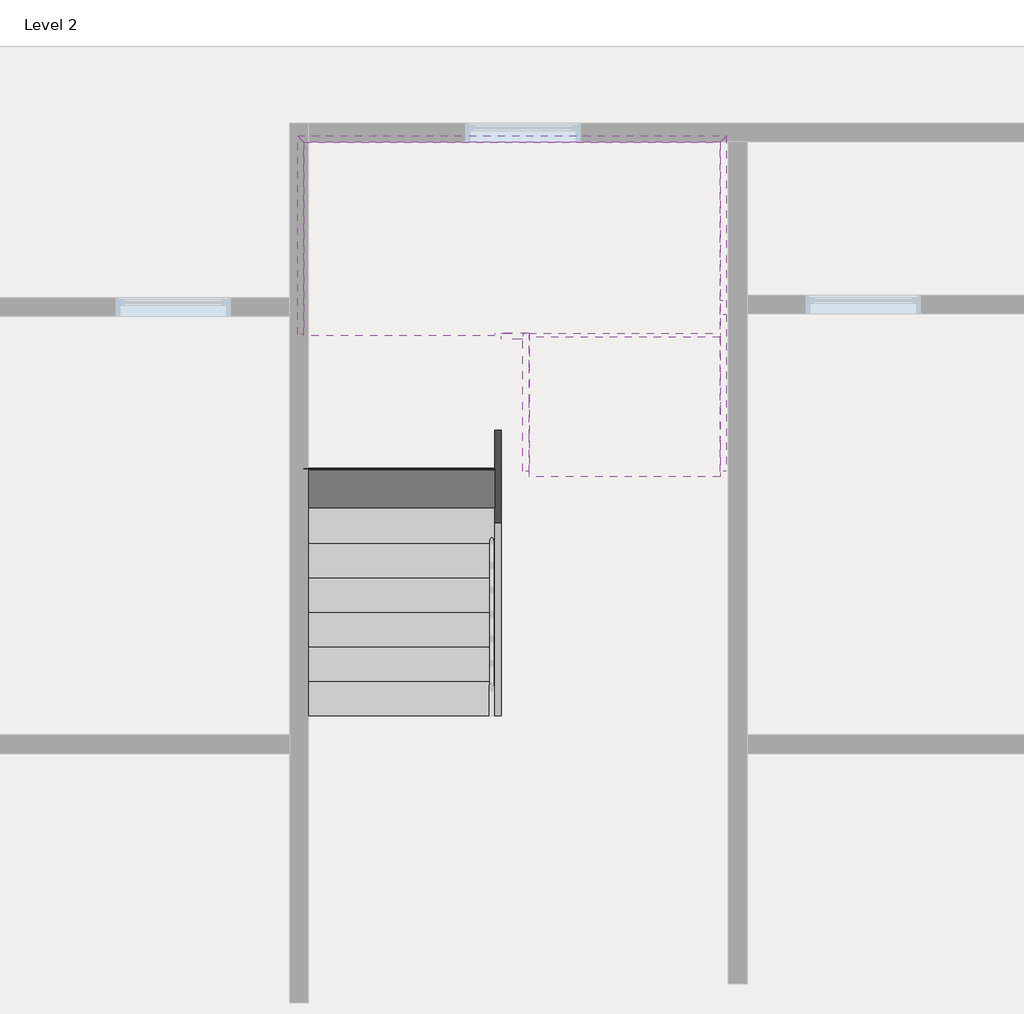
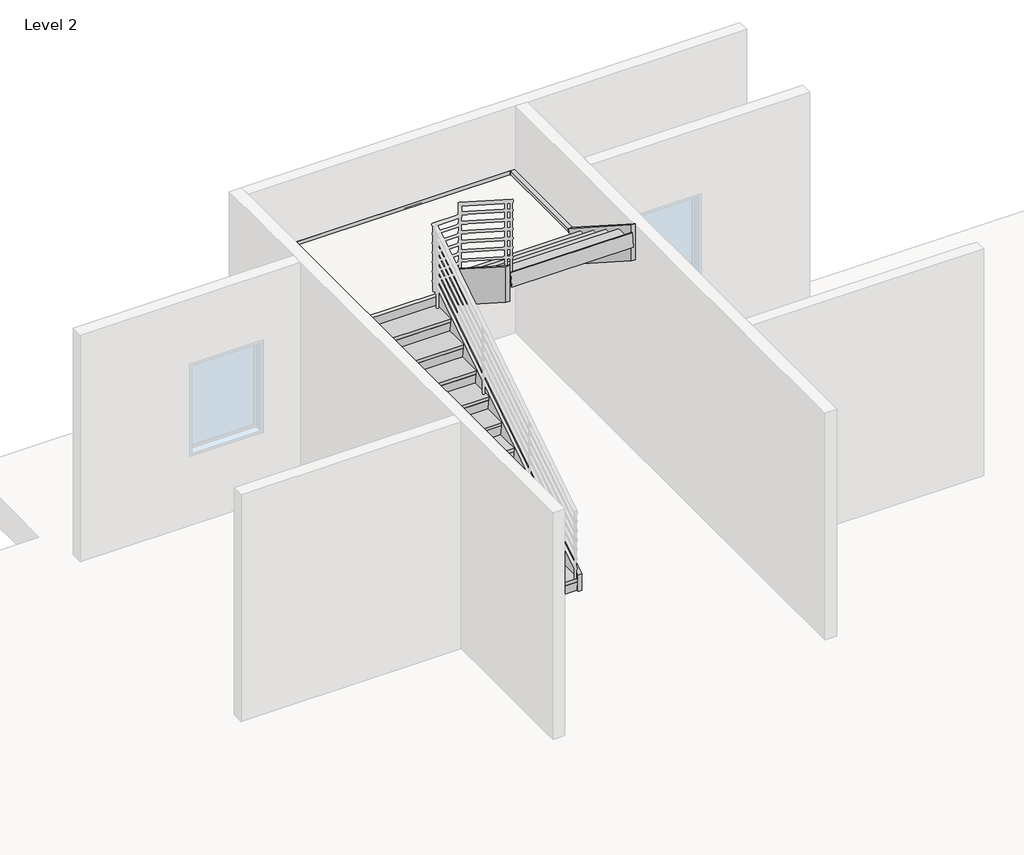
# One storey, part 7 of 7: 8 members, 2 stair flights, 1 slab.
"""IFC4 building model written with IfcOpenShell, lengths in millimetres."""

import ifcopenshell
import ifcopenshell.guid

model = None  # the IFC model being written
_history = None  # IfcOwnerHistory: only IFC2X3 demands one
_inside = {}  # id of a spatial element -> (the spatial element, [elements in it])
_under = {}  # id of a project, library or spatial element -> (it, [spatial elements below it])
_declared = {}  # id of a project -> (the project, [libraries it declares])
_typed = {}  # id of a type object -> (the type object, [elements of that type])
_made_of = {}  # id of a material, layer set ... -> (it, [elements and type objects made of it])


def new_model(schema):
    """Start an empty IFC model of exactly this schema.

    Asked for "IFC4X3", IfcOpenShell would pick the latest addendum, in which some entities
    have other attributes; the version numbers below select the first issue.
    IFC2X3 requires an IfcOwnerHistory on every rooted entity: one is made here for all.
    """
    global model, _history
    if schema == "IFC4X3":
        model = ifcopenshell.file(schema_version=(4, 3, 0, 0))
    else:
        model = ifcopenshell.file(schema=schema)
    _inside.clear()
    _under.clear()
    _declared.clear()
    _typed.clear()
    _made_of.clear()
    _history = None
    if model.schema == "IFC2X3":
        org = make("IfcOrganization", Name="unknown")
        user = make(
            "IfcPersonAndOrganization",
            ThePerson=make("IfcPerson", FamilyName="unknown"),
            TheOrganization=org,
        )
        app = make(
            "IfcApplication",
            ApplicationDeveloper=org,
            Version="unknown",
            ApplicationFullName="unknown",
            ApplicationIdentifier="unknown",
        )
        _history = make(
            "IfcOwnerHistory",
            OwningUser=user,
            OwningApplication=app,
            ChangeAction="ADDED",
            CreationDate=0,
        )
    return model


def make(cls, **values):
    """One entity of the class cls with the attributes given. An attribute that is None is left unset."""
    return model.create_entity(
        cls, **{name: value for name, value in values.items() if value is not None}
    )


def rooted(cls, **values):
    """An entity with a GlobalId (a new one), such as an element, a storey or a relation."""
    return make(cls, GlobalId=ifcopenshell.guid.new(), OwnerHistory=_history, **values)


def si_unit(unit_type, name, prefix=None):
    """IfcSIUnit, for example si_unit("LENGTHUNIT", "METRE", prefix="MILLI")."""
    return make("IfcSIUnit", UnitType=unit_type, Prefix=prefix, Name=name)


def assignment(units):
    """IfcUnitAssignment: the units of a project."""
    return None if units is None else make("IfcUnitAssignment", Units=units)


def point(xyz):
    """IfcCartesianPoint."""
    return None if xyz is None else make("IfcCartesianPoint", Coordinates=xyz)


def direction(xyz):
    """IfcDirection."""
    return None if xyz is None else make("IfcDirection", DirectionRatios=xyz)


def frame(location, z_axis=None, x_axis=None):
    """IfcAxis2Placement3D, a coordinate frame: its origin and axes. An axis left out is left unset."""
    return make(
        "IfcAxis2Placement3D",
        Location=point(location),
        Axis=direction(z_axis),
        RefDirection=direction(x_axis),
    )


def origin():
    """The frame at (0, 0, 0) with its axes left unset."""
    return frame((0.0, 0.0, 0.0))


def place(relative_to, where):
    """IfcLocalPlacement: puts the frame where relative to a parent placement (None: the world)."""
    return make(
        "IfcLocalPlacement", PlacementRelTo=relative_to, RelativePlacement=where
    )


def context(
    kind, dimensions, precision=None, world=None, true_north=None, identifier=None
):
    """IfcGeometricRepresentationContext, for example the 3D "Model" context."""
    return make(
        "IfcGeometricRepresentationContext",
        ContextIdentifier=identifier,
        ContextType=kind,
        CoordinateSpaceDimension=dimensions,
        Precision=precision,
        WorldCoordinateSystem=world,
        TrueNorth=true_north,
    )


def project(units=None, contexts=None):
    """IfcProject with its units and contexts."""
    return rooted(
        "IfcProject",
        Name="project",
        RepresentationContexts=contexts,
        UnitsInContext=assignment(units),
    )


def spatial(cls, under=None, at=None, **own):
    """A site, building, storey or space (cls), placed at a placement, below another one or the project."""
    s = rooted(cls, ObjectPlacement=at, **own)
    if under is not None:
        _under.setdefault(under.id(), (under, []))[1].append(s)
    return s


def polyline(points):
    """IfcPolyline through the points."""
    return make("IfcPolyline", Points=[point(p) for p in points])


def outline(outer, holes=None, kind="AREA"):
    """IfcArbitraryClosedProfileDef: a profile drawn as a closed curve; with holes, ...WithVoids."""
    if holes is None:
        return make("IfcArbitraryClosedProfileDef", ProfileType=kind, OuterCurve=outer)
    return make(
        "IfcArbitraryProfileDefWithVoids",
        ProfileType=kind,
        OuterCurve=outer,
        InnerCurves=holes,
    )


def extrude(swept, where, along, depth):
    """IfcExtrudedAreaSolid: the profile swept, set in the frame where, extruded along a direction by depth."""
    return make(
        "IfcExtrudedAreaSolid",
        SweptArea=swept,
        Position=where,
        ExtrudedDirection=direction(along),
        Depth=depth,
    )


def faces_of(points, faces, orient=None, outer=None):
    """IfcFace entities. A face is a list of loops; a loop is a list of indices into points, from 0.

    orient and outer hold one flag for each loop. By default every Orientation is true, the
    first loop of a face is its IfcFaceOuterBound and the others are IfcFaceBound.
    """
    made = []
    for i, loops in enumerate(faces):
        bounds = []
        for j, loop in enumerate(loops):
            is_outer = j == 0 if outer is None else outer[i][j]
            bounds.append(
                make(
                    "IfcFaceOuterBound" if is_outer else "IfcFaceBound",
                    Bound=make("IfcPolyLoop", Polygon=[points[k] for k in loop]),
                    Orientation=True if orient is None else orient[i][j],
                )
            )
        made.append(make("IfcFace", Bounds=bounds))
    return made


def faceted_brep(points, faces, orient=None, outer=None, voids=None):
    """IfcFacetedBrep: a solid bounded by flat faces; with voids (closed shells), ...WithVoids."""
    shared = [point(p) for p in points]
    hull = make("IfcClosedShell", CfsFaces=faces_of(shared, faces, orient, outer))
    if voids is None:
        return make("IfcFacetedBrep", Outer=hull)
    return make(
        "IfcFacetedBrepWithVoids",
        Outer=hull,
        Voids=[
            make(cls, CfsFaces=faces_of(shared, fs, o, b)) for cls, fs, o, b in voids
        ],
    )


def shape(context_of_items, identifier, shape_type, items):
    """IfcShapeRepresentation: the items that make up one representation, for example the "Body"."""
    return make(
        "IfcShapeRepresentation",
        ContextOfItems=context_of_items,
        RepresentationIdentifier=identifier,
        RepresentationType=shape_type,
        Items=items,
    )


def source(mapping_origin, context_of_items, identifier, shape_type, items):
    """IfcRepresentationMap: a shape defined once, which mapped items show again and again."""
    return make(
        "IfcRepresentationMap",
        MappingOrigin=mapping_origin,
        MappedRepresentation=shape(context_of_items, identifier, shape_type, items),
    )


def transform(
    local_origin,
    x_axis=None,
    y_axis=None,
    z_axis=None,
    scale=None,
    scale2=None,
    scale3=None,
    uniform=True,
):
    """IfcCartesianTransformationOperator3D, or its non-uniform kind. x_axis, y_axis, z_axis: its Axis1, 2, 3."""
    if uniform:
        return make(
            "IfcCartesianTransformationOperator3D",
            Axis1=direction(x_axis),
            Axis2=direction(y_axis),
            LocalOrigin=point(local_origin),
            Scale=scale,
            Axis3=direction(z_axis),
        )
    return make(
        "IfcCartesianTransformationOperator3DnonUniform",
        Axis1=direction(x_axis),
        Axis2=direction(y_axis),
        LocalOrigin=point(local_origin),
        Scale=scale,
        Axis3=direction(z_axis),
        Scale2=scale2,
        Scale3=scale3,
    )


def mapped(mapping_source, mapping_target):
    """IfcMappedItem: shows the shape of a source again, moved by a transform."""
    return make(
        "IfcMappedItem", MappingSource=mapping_source, MappingTarget=mapping_target
    )


def made_of(thing, what):
    """Note that an element or type object is made of a material, layer set ...; save() writes the relation."""
    if what is not None:
        _made_of.setdefault(what.id(), (what, []))[1].append(thing)
    return thing


def element(
    cls,
    number,
    at=None,
    inside=None,
    cuts=None,
    type_object=None,
    material=None,
    context=None,
    identifier="Body",
    shape_type=None,
    held_by="IfcProductDefinitionShape",
    body=None,
    shapes=None,
    **own,
):
    """One element of the class cls, such as IfcWall. Its Tag is "e" and its number.

    at: its placement. inside: the storey or other place that contains it. cuts: it is an
    opening in that element (IfcRelVoidsElement). A single representation is given by context,
    identifier, shape_type and body (its items); several are given by shapes. held_by: the class
    of the entity that holds the representations. save() writes the other relations.
    """
    e = rooted(cls, Tag="e%d" % number, ObjectPlacement=at, **own)
    if body is not None:
        shapes = [shape(context, identifier, shape_type, body)]
    if shapes is not None:
        e.Representation = make(held_by, Representations=shapes)
    if inside is not None:
        _inside.setdefault(inside.id(), (inside, []))[1].append(e)
    if cuts is not None:
        rooted(
            "IfcRelVoidsElement", RelatingBuildingElement=cuts, RelatedOpeningElement=e
        )
    if type_object is not None:
        _typed.setdefault(type_object.id(), (type_object, []))[1].append(e)
    return made_of(e, material)


def aggregate(whole, parts):
    """IfcRelAggregates: a whole, such as a stair, and the parts it consists of."""
    return rooted("IfcRelAggregates", RelatingObject=whole, RelatedObjects=parts)


def save(model, path):
    """Write the relations noted so far, then the file.

    IfcRelAggregates (storeys below a building ...), IfcRelContainedInSpatialStructure (elements
    in a storey), IfcRelDefinesByType, IfcRelAssociatesMaterial and IfcRelDeclares: one each for
    every whole, place, type object, material and project.
    """
    for whole, parts in _under.values():
        aggregate(whole, parts)
    for where, things in _inside.values():
        rooted(
            "IfcRelContainedInSpatialStructure",
            RelatedElements=things,
            RelatingStructure=where,
        )
    for kind, things in _typed.values():
        rooted("IfcRelDefinesByType", RelatedObjects=things, RelatingType=kind)
    for what, things in _made_of.values():
        rooted("IfcRelAssociatesMaterial", RelatedObjects=things, RelatingMaterial=what)
    for by, libraries in _declared.values():
        rooted("IfcRelDeclares", RelatingContext=by, RelatedDefinitions=libraries)
    model.write(path)


def non_monolithic_landing_3f935088(model_context):
    return source(origin(), model_context, "Body", "Brep", [
        faceted_brep([(-226.7120949, 7307.4781803, 5617.6470588), (-226.7120949, 7300.3948469, 5567.6470588), (1293.2879051, 7300.3948469, 5567.6470588), (1293.2879051, 7307.4781803, 5617.6470588), (-499.4393676, 7309.7509075, 5617.6470588), (-499.4393676, 7332.4781803, 5617.6470588), (-226.7120949, 7332.4781803, 5617.6470588), (1293.2879051, 7332.4781803, 5617.6470588), (1293.2879051, 8852.4781803, 5617.6470588), (-2019.4393676, 8852.4781803, 5617.6470588), (-2019.4393676, 7309.7509075, 5617.6470588), (-226.7120949, 7332.4781803, 5567.6470588), (-499.4393676, 7332.4781803, 5567.6470588), (-499.4393676, 7316.8342409, 5567.6470588), (-2019.4393676, 7316.8342409, 5567.6470588), (-2019.4393676, 8852.4781803, 5567.6470588), (1293.2879051, 8852.4781803, 5567.6470588), (1293.2879051, 7332.4781803, 5567.6470588)], [[[0, 1, 2, 3]], [[4, 5, 6, 0, 3, 7, 8, 9, 10]], [[11, 12, 13, 14, 15, 16, 17, 2, 1]], [[5, 4, 13, 12]], [[6, 5, 12, 11]], [[0, 6, 11, 1]], [[7, 3, 2, 17]], [[8, 7, 17, 16]], [[9, 8, 16, 15]], [[10, 9, 15, 14]], [[4, 10, 14, 13]]]),
    ])


def stair_flight_50mm_tread_25mm_nosing_13mm_riser_1a7390ad(model_context):
    return source(origin(), model_context, "Body", "Brep", [
        faceted_brep([(-499.4393676, 4584.7509075, 3676.4705882), (-499.4393676, 4591.8342409, 3626.4705882), (-2019.4393676, 4591.8342409, 3626.4705882), (-2019.4393676, 4584.7509075, 3676.4705882), (-2019.4393676, 4284.7509075, 3676.4705882), (-499.4393676, 4284.7509075, 3676.4705882), (-499.4393676, 4291.8342409, 3626.4705882), (-2019.4393676, 4291.8342409, 3626.4705882)], [[[0, 1, 2, 3]], [[3, 4, 5, 0]], [[2, 1, 6, 7]], [[4, 3, 2, 7]], [[0, 5, 6, 1]], [[5, 4, 7, 6]]]),
        faceted_brep([(-499.4393676, 4291.8342409, 3626.4705882), (-499.4393676, 4309.7509075, 3500.0), (-499.4393676, 4322.3757185, 3500.0), (-499.4393676, 4304.4590518, 3626.4705882), (-2019.4393676, 4291.8342409, 3626.4705882), (-2019.4393676, 4304.4590518, 3626.4705882), (-2019.4393676, 4322.3757185, 3500.0), (-2019.4393676, 4309.7509075, 3500.0)], [[[0, 1, 2, 3]], [[4, 5, 6, 7]], [[1, 0, 4, 7]], [[2, 1, 7, 6]], [[3, 2, 6, 5]], [[0, 3, 5, 4]]]),
        faceted_brep([(-499.4393676, 4566.8342409, 3802.9411765), (-499.4393676, 4591.8342409, 3626.4705882), (-499.4393676, 4604.4590518, 3626.4705882), (-499.4393676, 4579.4590518, 3802.9411765), (-2019.4393676, 4566.8342409, 3802.9411765), (-2019.4393676, 4579.4590518, 3802.9411765), (-2019.4393676, 4604.4590518, 3626.4705882), (-2019.4393676, 4591.8342409, 3626.4705882)], [[[0, 1, 2, 3]], [[4, 5, 6, 7]], [[1, 0, 4, 7]], [[2, 1, 7, 6]], [[3, 2, 6, 5]], [[0, 3, 5, 4]]]),
        faceted_brep([(-2019.4393676, 4859.7509075, 3852.9411765), (-2019.4393676, 4559.7509075, 3852.9411765), (-499.4393676, 4559.7509075, 3852.9411765), (-499.4393676, 4859.7509075, 3852.9411765), (-2019.4393676, 4866.8342409, 3802.9411765), (-499.4393676, 4866.8342409, 3802.9411765), (-499.4393676, 4566.8342409, 3802.9411765), (-2019.4393676, 4566.8342409, 3802.9411765)], [[[0, 1, 2, 3]], [[4, 5, 6, 7]], [[1, 0, 4, 7]], [[3, 2, 6, 5]], [[3, 5, 4, 0]], [[2, 1, 7, 6]]]),
        faceted_brep([(-499.4393676, 4841.8342409, 3979.4117647), (-499.4393676, 4866.8342409, 3802.9411765), (-499.4393676, 4879.4590518, 3802.9411765), (-499.4393676, 4854.4590518, 3979.4117647), (-2019.4393676, 4841.8342409, 3979.4117647), (-2019.4393676, 4854.4590518, 3979.4117647), (-2019.4393676, 4879.4590518, 3802.9411765), (-2019.4393676, 4866.8342409, 3802.9411765)], [[[0, 1, 2, 3]], [[4, 5, 6, 7]], [[1, 0, 4, 7]], [[2, 1, 7, 6]], [[3, 2, 6, 5]], [[0, 3, 5, 4]]]),
        faceted_brep([(-2019.4393676, 5134.7509075, 4029.4117647), (-2019.4393676, 4834.7509075, 4029.4117647), (-499.4393676, 4834.7509075, 4029.4117647), (-499.4393676, 5134.7509075, 4029.4117647), (-2019.4393676, 5141.8342409, 3979.4117647), (-499.4393676, 5141.8342409, 3979.4117647), (-499.4393676, 4841.8342409, 3979.4117647), (-2019.4393676, 4841.8342409, 3979.4117647)], [[[0, 1, 2, 3]], [[4, 5, 6, 7]], [[1, 0, 4, 7]], [[3, 2, 6, 5]], [[3, 5, 4, 0]], [[2, 1, 7, 6]]]),
        faceted_brep([(-499.4393676, 5116.8342409, 4155.8823529), (-499.4393676, 5141.8342409, 3979.4117647), (-499.4393676, 5154.4590518, 3979.4117647), (-499.4393676, 5129.4590518, 4155.8823529), (-2019.4393676, 5116.8342409, 4155.8823529), (-2019.4393676, 5129.4590518, 4155.8823529), (-2019.4393676, 5154.4590518, 3979.4117647), (-2019.4393676, 5141.8342409, 3979.4117647)], [[[0, 1, 2, 3]], [[4, 5, 6, 7]], [[1, 0, 4, 7]], [[2, 1, 7, 6]], [[3, 2, 6, 5]], [[0, 3, 5, 4]]]),
        faceted_brep([(-2019.4393676, 5409.7509075, 4205.8823529), (-2019.4393676, 5109.7509075, 4205.8823529), (-499.4393676, 5109.7509075, 4205.8823529), (-499.4393676, 5409.7509075, 4205.8823529), (-2019.4393676, 5416.8342409, 4155.8823529), (-499.4393676, 5416.8342409, 4155.8823529), (-499.4393676, 5116.8342409, 4155.8823529), (-2019.4393676, 5116.8342409, 4155.8823529)], [[[0, 1, 2, 3]], [[4, 5, 6, 7]], [[1, 0, 4, 7]], [[3, 2, 6, 5]], [[3, 5, 4, 0]], [[2, 1, 7, 6]]]),
        faceted_brep([(-499.4393676, 5391.8342409, 4332.3529412), (-499.4393676, 5416.8342409, 4155.8823529), (-499.4393676, 5429.4590518, 4155.8823529), (-499.4393676, 5404.4590518, 4332.3529412), (-2019.4393676, 5391.8342409, 4332.3529412), (-2019.4393676, 5404.4590518, 4332.3529412), (-2019.4393676, 5429.4590518, 4155.8823529), (-2019.4393676, 5416.8342409, 4155.8823529)], [[[0, 1, 2, 3]], [[4, 5, 6, 7]], [[1, 0, 4, 7]], [[2, 1, 7, 6]], [[3, 2, 6, 5]], [[0, 3, 5, 4]]]),
        faceted_brep([(-2019.4393676, 5684.7509075, 4382.3529412), (-2019.4393676, 5384.7509075, 4382.3529412), (-499.4393676, 5384.7509075, 4382.3529412), (-499.4393676, 5684.7509075, 4382.3529412), (-2019.4393676, 5691.8342409, 4332.3529412), (-499.4393676, 5691.8342409, 4332.3529412), (-499.4393676, 5391.8342409, 4332.3529412), (-2019.4393676, 5391.8342409, 4332.3529412)], [[[0, 1, 2, 3]], [[4, 5, 6, 7]], [[1, 0, 4, 7]], [[3, 2, 6, 5]], [[3, 5, 4, 0]], [[2, 1, 7, 6]]]),
        faceted_brep([(-499.4393676, 5666.8342409, 4508.8235294), (-499.4393676, 5691.8342409, 4332.3529412), (-499.4393676, 5704.4590518, 4332.3529412), (-499.4393676, 5679.4590518, 4508.8235294), (-2019.4393676, 5666.8342409, 4508.8235294), (-2019.4393676, 5679.4590518, 4508.8235294), (-2019.4393676, 5704.4590518, 4332.3529412), (-2019.4393676, 5691.8342409, 4332.3529412)], [[[0, 1, 2, 3]], [[4, 5, 6, 7]], [[1, 0, 4, 7]], [[2, 1, 7, 6]], [[3, 2, 6, 5]], [[0, 3, 5, 4]]]),
        faceted_brep([(-2019.4393676, 5959.7509075, 4558.8235294), (-2019.4393676, 5659.7509075, 4558.8235294), (-499.4393676, 5659.7509075, 4558.8235294), (-499.4393676, 5959.7509075, 4558.8235294), (-2019.4393676, 5966.8342409, 4508.8235294), (-499.4393676, 5966.8342409, 4508.8235294), (-499.4393676, 5666.8342409, 4508.8235294), (-2019.4393676, 5666.8342409, 4508.8235294)], [[[0, 1, 2, 3]], [[4, 5, 6, 7]], [[1, 0, 4, 7]], [[3, 2, 6, 5]], [[3, 5, 4, 0]], [[2, 1, 7, 6]]]),
        faceted_brep([(-499.4393676, 5941.8342409, 4685.2941176), (-499.4393676, 5966.8342409, 4508.8235294), (-499.4393676, 5979.4590518, 4508.8235294), (-499.4393676, 5954.4590518, 4685.2941176), (-2019.4393676, 5941.8342409, 4685.2941176), (-2019.4393676, 5954.4590518, 4685.2941176), (-2019.4393676, 5979.4590518, 4508.8235294), (-2019.4393676, 5966.8342409, 4508.8235294)], [[[0, 1, 2, 3]], [[4, 5, 6, 7]], [[1, 0, 4, 7]], [[2, 1, 7, 6]], [[3, 2, 6, 5]], [[0, 3, 5, 4]]]),
        faceted_brep([(-2019.4393676, 6234.7509075, 4735.2941176), (-2019.4393676, 5934.7509075, 4735.2941176), (-499.4393676, 5934.7509075, 4735.2941176), (-499.4393676, 6234.7509075, 4735.2941176), (-2019.4393676, 6241.8342409, 4685.2941176), (-499.4393676, 6241.8342409, 4685.2941176), (-499.4393676, 5941.8342409, 4685.2941176), (-2019.4393676, 5941.8342409, 4685.2941176)], [[[0, 1, 2, 3]], [[4, 5, 6, 7]], [[1, 0, 4, 7]], [[3, 2, 6, 5]], [[3, 5, 4, 0]], [[2, 1, 7, 6]]]),
        faceted_brep([(-499.4393676, 6216.8342409, 4861.7647059), (-499.4393676, 6241.8342409, 4685.2941176), (-499.4393676, 6254.4590518, 4685.2941176), (-499.4393676, 6229.4590518, 4861.7647059), (-2019.4393676, 6216.8342409, 4861.7647059), (-2019.4393676, 6229.4590518, 4861.7647059), (-2019.4393676, 6254.4590518, 4685.2941176), (-2019.4393676, 6241.8342409, 4685.2941176)], [[[0, 1, 2, 3]], [[4, 5, 6, 7]], [[1, 0, 4, 7]], [[2, 1, 7, 6]], [[3, 2, 6, 5]], [[0, 3, 5, 4]]]),
        faceted_brep([(-2019.4393676, 6509.7509075, 4911.7647059), (-2019.4393676, 6209.7509075, 4911.7647059), (-499.4393676, 6209.7509075, 4911.7647059), (-499.4393676, 6509.7509075, 4911.7647059), (-2019.4393676, 6516.8342409, 4861.7647059), (-499.4393676, 6516.8342409, 4861.7647059), (-499.4393676, 6216.8342409, 4861.7647059), (-2019.4393676, 6216.8342409, 4861.7647059)], [[[0, 1, 2, 3]], [[4, 5, 6, 7]], [[1, 0, 4, 7]], [[3, 2, 6, 5]], [[3, 5, 4, 0]], [[2, 1, 7, 6]]]),
        faceted_brep([(-499.4393676, 6491.8342409, 5038.2352941), (-499.4393676, 6516.8342409, 4861.7647059), (-499.4393676, 6529.4590518, 4861.7647059), (-499.4393676, 6504.4590518, 5038.2352941), (-2019.4393676, 6491.8342409, 5038.2352941), (-2019.4393676, 6504.4590518, 5038.2352941), (-2019.4393676, 6529.4590518, 4861.7647059), (-2019.4393676, 6516.8342409, 4861.7647059)], [[[0, 1, 2, 3]], [[4, 5, 6, 7]], [[1, 0, 4, 7]], [[2, 1, 7, 6]], [[3, 2, 6, 5]], [[0, 3, 5, 4]]]),
        faceted_brep([(-2019.4393676, 6784.7509075, 5088.2352941), (-2019.4393676, 6484.7509075, 5088.2352941), (-499.4393676, 6484.7509075, 5088.2352941), (-499.4393676, 6784.7509075, 5088.2352941), (-2019.4393676, 6791.8342409, 5038.2352941), (-499.4393676, 6791.8342409, 5038.2352941), (-499.4393676, 6491.8342409, 5038.2352941), (-2019.4393676, 6491.8342409, 5038.2352941)], [[[0, 1, 2, 3]], [[4, 5, 6, 7]], [[1, 0, 4, 7]], [[3, 2, 6, 5]], [[3, 5, 4, 0]], [[2, 1, 7, 6]]]),
        faceted_brep([(-499.4393676, 6766.8342409, 5214.7058824), (-499.4393676, 6791.8342409, 5038.2352941), (-499.4393676, 6804.4590518, 5038.2352941), (-499.4393676, 6779.4590518, 5214.7058824), (-2019.4393676, 6766.8342409, 5214.7058824), (-2019.4393676, 6779.4590518, 5214.7058824), (-2019.4393676, 6804.4590518, 5038.2352941), (-2019.4393676, 6791.8342409, 5038.2352941)], [[[0, 1, 2, 3]], [[4, 5, 6, 7]], [[1, 0, 4, 7]], [[2, 1, 7, 6]], [[3, 2, 6, 5]], [[0, 3, 5, 4]]]),
        faceted_brep([(-2019.4393676, 7059.7509075, 5264.7058824), (-2019.4393676, 6759.7509075, 5264.7058824), (-499.4393676, 6759.7509075, 5264.7058824), (-499.4393676, 7059.7509075, 5264.7058824), (-2019.4393676, 7066.8342409, 5214.7058824), (-499.4393676, 7066.8342409, 5214.7058824), (-499.4393676, 6766.8342409, 5214.7058824), (-2019.4393676, 6766.8342409, 5214.7058824)], [[[0, 1, 2, 3]], [[4, 5, 6, 7]], [[1, 0, 4, 7]], [[3, 2, 6, 5]], [[3, 5, 4, 0]], [[2, 1, 7, 6]]]),
        faceted_brep([(-499.4393676, 7316.8342409, 5567.6470588), (-499.4393676, 7341.8342409, 5391.1764706), (-499.4393676, 7354.4590518, 5391.1764706), (-499.4393676, 7329.4590518, 5567.6470588), (-2019.4393676, 7316.8342409, 5567.6470588), (-2019.4393676, 7329.4590518, 5567.6470588), (-2019.4393676, 7354.4590518, 5391.1764706), (-2019.4393676, 7341.8342409, 5391.1764706)], [[[0, 1, 2, 3]], [[4, 5, 6, 7]], [[1, 0, 4, 7]], [[2, 1, 7, 6]], [[3, 2, 6, 5]], [[0, 3, 5, 4]]]),
        faceted_brep([(-499.4393676, 7041.8342409, 5391.1764706), (-499.4393676, 7066.8342409, 5214.7058824), (-499.4393676, 7079.4590518, 5214.7058824), (-499.4393676, 7054.4590518, 5391.1764706), (-2019.4393676, 7041.8342409, 5391.1764706), (-2019.4393676, 7054.4590518, 5391.1764706), (-2019.4393676, 7079.4590518, 5214.7058824), (-2019.4393676, 7066.8342409, 5214.7058824)], [[[0, 1, 2, 3]], [[4, 5, 6, 7]], [[1, 0, 4, 7]], [[2, 1, 7, 6]], [[3, 2, 6, 5]], [[0, 3, 5, 4]]]),
        faceted_brep([(-2019.4393676, 7334.7509075, 5441.1764706), (-2019.4393676, 7309.7509075, 5441.1764706), (-2019.4393676, 7034.7509075, 5441.1764706), (-499.4393676, 7034.7509075, 5441.1764706), (-499.4393676, 7334.7509075, 5441.1764706), (-2019.4393676, 7341.8342409, 5391.1764706), (-499.4393676, 7341.8342409, 5391.1764706), (-499.4393676, 7041.8342409, 5391.1764706), (-2019.4393676, 7041.8342409, 5391.1764706), (-2019.4393676, 7309.7509075, 5391.1764706)], [[[0, 1, 2, 3, 4]], [[5, 6, 7, 8, 9]], [[1, 0, 5, 9]], [[2, 1, 9, 8]], [[4, 3, 7, 6]], [[4, 6, 5, 0]], [[3, 2, 8, 7]]]),
    ])


def stair_flight_50mm_tread_25mm_nosing_13mm_riser_b21a55c2(model_context):
    return source(origin(), model_context, "Body", "SweptSolid", [
        extrude(outline(polyline([(7032.4781803, 5794.1176471), (7332.4781803, 5794.1176471), (7325.3948469, 5744.1176471), (7025.3948469, 5744.1176471), (7032.4781803, 5794.1176471)])), frame((-226.7120949, 0.0, 0.0), z_axis=(1.0, 0.0, 0.0), x_axis=(0.0, 1.0, 0.0)), (0.0, 0.0, 1.0), 1520.0),
        extrude(outline(polyline([(7325.3948469, 5744.1176471), (7300.3948469, 5567.6470588), (7287.770036, 5567.6470588), (7312.770036, 5744.1176471), (7325.3948469, 5744.1176471)])), frame((-226.7120949, 0.0, 0.0), z_axis=(1.0, 0.0, 0.0), x_axis=(0.0, 1.0, 0.0)), (0.0, 0.0, 1.0), 1520.0),
        extrude(outline(polyline([(7050.3948469, 5920.5882353), (7025.3948469, 5744.1176471), (7012.770036, 5744.1176471), (7037.770036, 5920.5882353), (7050.3948469, 5920.5882353)])), frame((-226.7120949, 0.0, 0.0), z_axis=(1.0, 0.0, 0.0), x_axis=(0.0, 1.0, 0.0)), (0.0, 0.0, 1.0), 1520.0),
        extrude(outline(polyline([(6757.4781803, 5970.5882353), (7057.4781803, 5970.5882353), (7050.3948469, 5920.5882353), (6750.3948469, 5920.5882353), (6757.4781803, 5970.5882353)])), frame((-226.7120949, 0.0, 0.0), z_axis=(1.0, 0.0, 0.0), x_axis=(0.0, 1.0, 0.0)), (0.0, 0.0, 1.0), 1520.0),
        extrude(outline(polyline([(6775.3948469, 6097.0588235), (6750.3948469, 5920.5882353), (6737.770036, 5920.5882353), (6762.770036, 6097.0588235), (6775.3948469, 6097.0588235)])), frame((-226.7120949, 0.0, 0.0), z_axis=(1.0, 0.0, 0.0), x_axis=(0.0, 1.0, 0.0)), (0.0, 0.0, 1.0), 1520.0),
        extrude(outline(polyline([(6482.4781803, 6147.0588235), (6782.4781803, 6147.0588235), (6775.3948469, 6097.0588235), (6475.3948469, 6097.0588235), (6482.4781803, 6147.0588235)])), frame((-226.7120949, 0.0, 0.0), z_axis=(1.0, 0.0, 0.0), x_axis=(0.0, 1.0, 0.0)), (0.0, 0.0, 1.0), 1520.0),
        extrude(outline(polyline([(6500.3948469, 6273.5294118), (6475.3948469, 6097.0588235), (6462.770036, 6097.0588235), (6487.770036, 6273.5294118), (6500.3948469, 6273.5294118)])), frame((-226.7120949, 0.0, 0.0), z_axis=(1.0, 0.0, 0.0), x_axis=(0.0, 1.0, 0.0)), (0.0, 0.0, 1.0), 1520.0),
        extrude(outline(polyline([(6225.3948469, 6450.0), (6200.3948469, 6273.5294118), (6187.770036, 6273.5294118), (6212.770036, 6450.0), (6225.3948469, 6450.0)])), frame((-226.7120949, 0.0, 0.0), z_axis=(1.0, 0.0, 0.0), x_axis=(0.0, 1.0, 0.0)), (0.0, 0.0, 1.0), 1520.0),
        extrude(outline(polyline([(6207.4781803, 6323.5294118), (6507.4781803, 6323.5294118), (6500.3948469, 6273.5294118), (6200.3948469, 6273.5294118), (6207.4781803, 6323.5294118)])), frame((-226.7120949, 0.0, 0.0), z_axis=(1.0, 0.0, 0.0), x_axis=(0.0, 1.0, 0.0)), (0.0, 0.0, 1.0), 1520.0),
    ])


model = new_model("IFC4")

# Units and contexts
model_context = context("Model", 3, world=origin())
ifc_project = project(units=[si_unit("LENGTHUNIT", "METRE", prefix="MILLI")], contexts=[model_context])

# Site, building, storey
site = spatial("IfcSite", under=ifc_project)
building = spatial("IfcBuilding", under=site)
storey = spatial("IfcBuildingStorey", under=building, Name="Level 2", Elevation=3500.0)

# Members
placement = place(None, origin())
element("IfcMember", 1, ObjectType="Stringer - 50mm Width", at=placement, inside=storey, context=model_context, shape_type="SweptSolid", body=[
    extrude(outline(polyline([(4284.7509075, 3500.0), (4284.7509075, 3715.9811749), (7322.0354678, 5665.0407858), (7439.3399977, 5265.0407858), (4688.8181065, 3500.0), (4284.7509075, 3500.0)])), frame((-2069.4393676, 0.0, 0.0), z_axis=(1.0, 0.0, 0.0), x_axis=(0.0, 1.0, 0.0)), (0.0, 0.0, 1.0), 50.0),
])
element("IfcMember", 2, ObjectType="Stringer - 50mm Width", at=placement, inside=storey, context=model_context, shape_type="SweptSolid", body=[
    extrude(outline(polyline([(4284.7509075, 3500.0), (4284.7509075, 3715.9811749), (7322.0354678, 5665.0407858), (7332.4781803, 5665.0407858), (7332.4781803, 5196.4663575), (4688.8181065, 3500.0), (4284.7509075, 3500.0)])), frame((-499.4393676, 0.0, 0.0), z_axis=(1.0, 0.0, 0.0), x_axis=(0.0, 1.0, 0.0)), (0.0, 0.0, 1.0), 50.0),
])
element("IfcMember", 3, ObjectType="Stringer - 50mm Width", at=placement, inside=storey, context=model_context, shape_type="SweptSolid", body=[
    extrude(outline(polyline([(7595.19362, 5665.0407858), (7477.8890902, 5265.0407858), (6232.4781803, 6064.2349525), (6232.4781803, 6539.5105867), (7595.19362, 5665.0407858)])), frame((1293.2879051, 0.0, 0.0), z_axis=(1.0, 0.0, 0.0), x_axis=(0.0, 1.0, 0.0)), (0.0, 0.0, 1.0), 50.0),
])
element("IfcMember", 4, ObjectType="Stringer - 50mm Width", at=placement, inside=storey, context=model_context, shape_type="SweptSolid", body=[
    extrude(outline(polyline([(7332.4781803, 5833.6282338), (7332.4781803, 5358.3525996), (6232.4781803, 6064.2349525), (6232.4781803, 6539.5105867), (7332.4781803, 5833.6282338)])), frame((-276.7120949, 0.0, 0.0), z_axis=(1.0, 0.0, 0.0), x_axis=(0.0, 1.0, 0.0)), (0.0, 0.0, 1.0), 50.0),
])
element("IfcMember", 5, ObjectType="Stringer - 50mm Width", at=placement, inside=storey, context=model_context, shape_type="Brep", body=[
    faceted_brep([(1293.2879051, 7595.19362, 5665.0407858), (1343.2879051, 7595.19362, 5665.0407858), (1343.2879051, 8902.4781803, 5665.0407858), (1293.2879051, 8852.4781803, 5665.0407858), (1293.2879051, 7477.8890902, 5265.0407858), (1293.2879051, 8852.4781803, 5265.0407858), (1343.2879051, 7477.8890902, 5265.0407858), (1343.2879051, 8902.4781803, 5265.0407858)], [[[0, 1, 2, 3]], [[4, 0, 3, 5]], [[6, 4, 5, 7]], [[1, 6, 7, 2]], [[1, 0, 4, 6]], [[2, 7, 5, 3]]]),
])
element("IfcMember", 6, ObjectType="Stringer - 50mm Width", at=placement, inside=storey, context=model_context, shape_type="SweptSolid", body=[
    extrude(outline(polyline([(1343.2879051, 8902.4781803), (1293.2879051, 8852.4781803), (-2019.4393676, 8852.4781803), (-2069.4393676, 8902.4781803), (1343.2879051, 8902.4781803)])), frame((0.0, 0.0, 5265.0407858), z_axis=(0.0, 0.0, 1.0), x_axis=(1.0, 0.0, 0.0)), (0.0, 0.0, 1.0), 400.0),
])
element("IfcMember", 7, ObjectType="Stringer - 50mm Width", at=placement, inside=storey, context=model_context, shape_type="Brep", body=[
    faceted_brep([(-2019.4393676, 8852.4781803, 5665.0407858), (-2069.4393676, 8902.4781803, 5665.0407858), (-2069.4393676, 7322.0354678, 5665.0407858), (-2019.4393676, 7322.0354678, 5665.0407858), (-2019.4393676, 8852.4781803, 5265.0407858), (-2019.4393676, 7439.3399977, 5265.0407858), (-2069.4393676, 8902.4781803, 5265.0407858), (-2069.4393676, 7439.3399977, 5265.0407858)], [[[0, 1, 2, 3]], [[4, 0, 3, 5]], [[6, 4, 5, 7]], [[1, 6, 7, 2]], [[1, 0, 4, 6]], [[2, 7, 5, 3]]]),
])
element("IfcMember", 8, ObjectType="Stringer - 50mm Width", at=placement, inside=storey, context=model_context, shape_type="SweptSolid", body=[
    extrude(outline(polyline([(-449.4393676, 7282.4781803), (-449.4393676, 7332.4781803), (-276.7120949, 7332.4781803), (-276.7120949, 7282.4781803), (-449.4393676, 7282.4781803)])), frame((0.0, 0.0, 5265.0407858), z_axis=(0.0, 0.0, 1.0), x_axis=(1.0, 0.0, 0.0)), (0.0, 0.0, 1.0), 400.0),
])

# Slab
non_monolithic_landing_shape = non_monolithic_landing_3f935088(model_context)
element("IfcSlab", 9, ObjectType="Non-Monolithic Landing", at=placement, inside=storey, context=model_context, shape_type="MappedRepresentation", body=[
    mapped(non_monolithic_landing_shape, transform((0.0, 0.0, 0.0), x_axis=(1.0, 0.0, 0.0), y_axis=(0.0, 1.0, 0.0), z_axis=(0.0, 0.0, 1.0))),
])

# Stair flights
stair_flight_50mm_tread_25mm_nosing_13mm_riser_shape = stair_flight_50mm_tread_25mm_nosing_13mm_riser_1a7390ad(model_context)
element("IfcStairFlight", 10, ObjectType="50mm Tread 25mm Nosing 13mm Riser", at=placement, inside=storey, context=model_context, shape_type="MappedRepresentation", body=[
    mapped(stair_flight_50mm_tread_25mm_nosing_13mm_riser_shape, transform((0.0, 0.0, 0.0), x_axis=(1.0, 0.0, 0.0), y_axis=(0.0, 1.0, 0.0), z_axis=(0.0, 0.0, 1.0))),
])
stair_flight_50mm_tread_25mm_nosing_13mm_riser_2_shape = stair_flight_50mm_tread_25mm_nosing_13mm_riser_b21a55c2(model_context)
element("IfcStairFlight", 11, ObjectType="50mm Tread 25mm Nosing 13mm Riser", at=placement, inside=storey, context=model_context, shape_type="MappedRepresentation", body=[
    mapped(stair_flight_50mm_tread_25mm_nosing_13mm_riser_2_shape, transform((0.0, 0.0, 0.0), x_axis=(1.0, 0.0, 0.0), y_axis=(0.0, 1.0, 0.0), z_axis=(0.0, 0.0, 1.0))),
])

save(model, "model.ifc")

# Revit data of these elements
# Elements 1, 2, 3, 4, 5, 6, 7, 8 (IfcMember, "Stringer - 50mm Width")
#   Phase Created = New Construction
# Element 9 (IfcSlab, "Non-Monolithic Landing")
#   Phase Created = New Construction
# Elements 10, 11 (IfcStairFlight, "50mm Tread 25mm Nosing 13mm Riser")
#   Phase Created = New Construction
